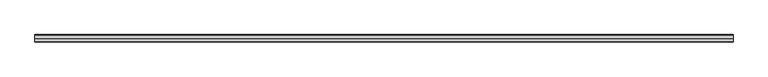
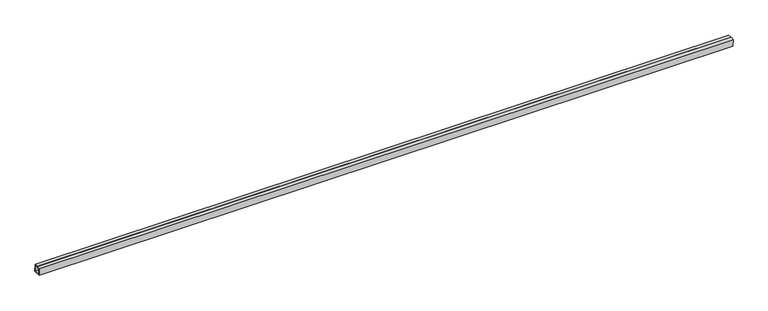
"""IFC4 building model written with IfcOpenShell, lengths in millimetres: proxy geometry, Inner panel:Inner panel:1:Inner panel:1 : Inner panel:Inner panel:300324:2:Inner panel:1:Inner panel:1 : Inner panel:Inner panel:300324:2 : Inner panel:Inner panel:1:Inner panel:1 : Inner panel:Inner panel:300324:300043:2 : Inner panel:Inner panel:1:Inner panel:1 : Inner panel:Inner panel:300324:2:Inner panel:1:Inner panel:1 : Inner panel:Inner panel:300324:2 : Inner panel:Inner panel:1:Inner panel:1 : Inner panel:Inner panel:300324:300043:308120."""

import ifcopenshell
import ifcopenshell.guid

model = None  # the IFC model being written
_history = None  # IfcOwnerHistory: only IFC2X3 demands one
_inside = {}  # id of a spatial element -> (the spatial element, [elements in it])
_under = {}  # id of a project, library or spatial element -> (it, [spatial elements below it])
_declared = {}  # id of a project -> (the project, [libraries it declares])
_typed = {}  # id of a type object -> (the type object, [elements of that type])
_made_of = {}  # id of a material, layer set ... -> (it, [elements and type objects made of it])


def new_model(schema):
    """Start an empty IFC model of exactly this schema.

    Asked for "IFC4X3", IfcOpenShell would pick the latest addendum, in which some entities
    have other attributes; the version numbers below select the first issue.
    IFC2X3 requires an IfcOwnerHistory on every rooted entity: one is made here for all.
    """
    global model, _history
    if schema == "IFC4X3":
        model = ifcopenshell.file(schema_version=(4, 3, 0, 0))
    else:
        model = ifcopenshell.file(schema=schema)
    _inside.clear()
    _under.clear()
    _declared.clear()
    _typed.clear()
    _made_of.clear()
    _history = None
    if model.schema == "IFC2X3":
        org = make("IfcOrganization", Name="unknown")
        user = make(
            "IfcPersonAndOrganization",
            ThePerson=make("IfcPerson", FamilyName="unknown"),
            TheOrganization=org,
        )
        app = make(
            "IfcApplication",
            ApplicationDeveloper=org,
            Version="unknown",
            ApplicationFullName="unknown",
            ApplicationIdentifier="unknown",
        )
        _history = make(
            "IfcOwnerHistory",
            OwningUser=user,
            OwningApplication=app,
            ChangeAction="ADDED",
            CreationDate=0,
        )
    return model


def make(cls, **values):
    """One entity of the class cls with the attributes given. An attribute that is None is left unset."""
    return model.create_entity(
        cls, **{name: value for name, value in values.items() if value is not None}
    )


def rooted(cls, **values):
    """An entity with a GlobalId (a new one), such as an element, a storey or a relation."""
    return make(cls, GlobalId=ifcopenshell.guid.new(), OwnerHistory=_history, **values)


def si_unit(unit_type, name, prefix=None):
    """IfcSIUnit, for example si_unit("LENGTHUNIT", "METRE", prefix="MILLI")."""
    return make("IfcSIUnit", UnitType=unit_type, Prefix=prefix, Name=name)


def assignment(units):
    """IfcUnitAssignment: the units of a project."""
    return None if units is None else make("IfcUnitAssignment", Units=units)


def point(xyz):
    """IfcCartesianPoint."""
    return None if xyz is None else make("IfcCartesianPoint", Coordinates=xyz)


def direction(xyz):
    """IfcDirection."""
    return None if xyz is None else make("IfcDirection", DirectionRatios=xyz)


def frame(location, z_axis=None, x_axis=None):
    """IfcAxis2Placement3D, a coordinate frame: its origin and axes. An axis left out is left unset."""
    return make(
        "IfcAxis2Placement3D",
        Location=point(location),
        Axis=direction(z_axis),
        RefDirection=direction(x_axis),
    )


def origin():
    """The frame at (0, 0, 0) with its axes left unset."""
    return frame((0.0, 0.0, 0.0))


def place(relative_to, where):
    """IfcLocalPlacement: puts the frame where relative to a parent placement (None: the world)."""
    return make(
        "IfcLocalPlacement", PlacementRelTo=relative_to, RelativePlacement=where
    )


def context(
    kind, dimensions, precision=None, world=None, true_north=None, identifier=None
):
    """IfcGeometricRepresentationContext, for example the 3D "Model" context."""
    return make(
        "IfcGeometricRepresentationContext",
        ContextIdentifier=identifier,
        ContextType=kind,
        CoordinateSpaceDimension=dimensions,
        Precision=precision,
        WorldCoordinateSystem=world,
        TrueNorth=true_north,
    )


def project(units=None, contexts=None):
    """IfcProject with its units and contexts."""
    return rooted(
        "IfcProject",
        Name="project",
        RepresentationContexts=contexts,
        UnitsInContext=assignment(units),
    )


def spatial(cls, under=None, at=None, **own):
    """A site, building, storey or space (cls), placed at a placement, below another one or the project."""
    s = rooted(cls, ObjectPlacement=at, **own)
    if under is not None:
        _under.setdefault(under.id(), (under, []))[1].append(s)
    return s


def polyline(points):
    """IfcPolyline through the points."""
    return make("IfcPolyline", Points=[point(p) for p in points])


def outline(outer, holes=None, kind="AREA"):
    """IfcArbitraryClosedProfileDef: a profile drawn as a closed curve; with holes, ...WithVoids."""
    if holes is None:
        return make("IfcArbitraryClosedProfileDef", ProfileType=kind, OuterCurve=outer)
    return make(
        "IfcArbitraryProfileDefWithVoids",
        ProfileType=kind,
        OuterCurve=outer,
        InnerCurves=holes,
    )


def extrude(swept, where, along, depth):
    """IfcExtrudedAreaSolid: the profile swept, set in the frame where, extruded along a direction by depth."""
    return make(
        "IfcExtrudedAreaSolid",
        SweptArea=swept,
        Position=where,
        ExtrudedDirection=direction(along),
        Depth=depth,
    )


def shape(context_of_items, identifier, shape_type, items):
    """IfcShapeRepresentation: the items that make up one representation, for example the "Body"."""
    return make(
        "IfcShapeRepresentation",
        ContextOfItems=context_of_items,
        RepresentationIdentifier=identifier,
        RepresentationType=shape_type,
        Items=items,
    )


def source(mapping_origin, context_of_items, identifier, shape_type, items):
    """IfcRepresentationMap: a shape defined once, which mapped items show again and again."""
    return make(
        "IfcRepresentationMap",
        MappingOrigin=mapping_origin,
        MappedRepresentation=shape(context_of_items, identifier, shape_type, items),
    )


def transform(
    local_origin,
    x_axis=None,
    y_axis=None,
    z_axis=None,
    scale=None,
    scale2=None,
    scale3=None,
    uniform=True,
):
    """IfcCartesianTransformationOperator3D, or its non-uniform kind. x_axis, y_axis, z_axis: its Axis1, 2, 3."""
    if uniform:
        return make(
            "IfcCartesianTransformationOperator3D",
            Axis1=direction(x_axis),
            Axis2=direction(y_axis),
            LocalOrigin=point(local_origin),
            Scale=scale,
            Axis3=direction(z_axis),
        )
    return make(
        "IfcCartesianTransformationOperator3DnonUniform",
        Axis1=direction(x_axis),
        Axis2=direction(y_axis),
        LocalOrigin=point(local_origin),
        Scale=scale,
        Axis3=direction(z_axis),
        Scale2=scale2,
        Scale3=scale3,
    )


def mapped(mapping_source, mapping_target):
    """IfcMappedItem: shows the shape of a source again, moved by a transform."""
    return make(
        "IfcMappedItem", MappingSource=mapping_source, MappingTarget=mapping_target
    )


def made_of(thing, what):
    """Note that an element or type object is made of a material, layer set ...; save() writes the relation."""
    if what is not None:
        _made_of.setdefault(what.id(), (what, []))[1].append(thing)
    return thing


def element(
    cls,
    number,
    at=None,
    inside=None,
    cuts=None,
    type_object=None,
    material=None,
    context=None,
    identifier="Body",
    shape_type=None,
    held_by="IfcProductDefinitionShape",
    body=None,
    shapes=None,
    **own,
):
    """One element of the class cls, such as IfcWall. Its Tag is "e" and its number.

    at: its placement. inside: the storey or other place that contains it. cuts: it is an
    opening in that element (IfcRelVoidsElement). A single representation is given by context,
    identifier, shape_type and body (its items); several are given by shapes. held_by: the class
    of the entity that holds the representations. save() writes the other relations.
    """
    e = rooted(cls, Tag="e%d" % number, ObjectPlacement=at, **own)
    if body is not None:
        shapes = [shape(context, identifier, shape_type, body)]
    if shapes is not None:
        e.Representation = make(held_by, Representations=shapes)
    if inside is not None:
        _inside.setdefault(inside.id(), (inside, []))[1].append(e)
    if cuts is not None:
        rooted(
            "IfcRelVoidsElement", RelatingBuildingElement=cuts, RelatedOpeningElement=e
        )
    if type_object is not None:
        _typed.setdefault(type_object.id(), (type_object, []))[1].append(e)
    return made_of(e, material)


def aggregate(whole, parts):
    """IfcRelAggregates: a whole, such as a stair, and the parts it consists of."""
    return rooted("IfcRelAggregates", RelatingObject=whole, RelatedObjects=parts)


def save(model, path):
    """Write the relations noted so far, then the file.

    IfcRelAggregates (storeys below a building ...), IfcRelContainedInSpatialStructure (elements
    in a storey), IfcRelDefinesByType, IfcRelAssociatesMaterial and IfcRelDeclares: one each for
    every whole, place, type object, material and project.
    """
    for whole, parts in _under.values():
        aggregate(whole, parts)
    for where, things in _inside.values():
        rooted(
            "IfcRelContainedInSpatialStructure",
            RelatedElements=things,
            RelatingStructure=where,
        )
    for kind, things in _typed.values():
        rooted("IfcRelDefinesByType", RelatedObjects=things, RelatingType=kind)
    for what, things in _made_of.values():
        rooted("IfcRelAssociatesMaterial", RelatedObjects=things, RelatingMaterial=what)
    for by, libraries in _declared.values():
        rooted("IfcRelDeclares", RelatingContext=by, RelatedDefinitions=libraries)
    model.write(path)


def generic_models_22e957f1(model_context):
    return source(origin(), model_context, "Body", "SweptSolid", [
        extrude(outline(polyline([(-579878.6983883, 3913.3147263), (-579860.4579651, 3914.0747439), (-579858.8718413, 3876.0077738), (-579896.9388114, 3874.4216501), (-579898.5249352, 3912.4886201), (-579880.284512, 3913.2486378), (-579880.1853793, 3910.8694521), (-579896.0466168, 3910.2085672), (-579894.6587585, 3876.8999684), (-579861.3501597, 3878.2878267), (-579862.738018, 3911.5964255), (-579878.5992555, 3910.9355406), (-579878.6983883, 3913.3147263)])), frame((593141.1867239, 0.0, 0.0), z_axis=(1.0, 0.0, 0.0), x_axis=(0.0, 1.0, 0.0)), (0.0, 0.0, 1.0), 3657.6),
    ])


if __name__ == "__main__":
    model = new_model("IFC4")
    model_context = context("Model", 3, world=origin())
    ifc_project = project(units=[si_unit("LENGTHUNIT", "METRE", prefix="MILLI")], contexts=[model_context])
    site = spatial("IfcSite", under=ifc_project)
    building = spatial("IfcBuilding", under=site)
    placement = place(None, origin())
    generic_models_shape = generic_models_22e957f1(model_context)
    element("IfcBuildingElementProxy", 1, Name="Inner panel:Inner panel:1:Inner panel:1 : Inner panel:Inner panel:300324:2:Inner panel:1:Inner panel:1 : Inner panel:Inner panel:300324:2 : Inner panel:Inner panel:1:Inner panel:1 : Inner panel:Inner panel:300324:300043:2 : Inner panel:Inner panel:1:Inner panel:1 : Inner panel:Inner panel:300324:2:Inner panel:1:Inner panel:1 : Inner panel:Inner panel:300324:2 : Inner panel:Inner panel:1:Inner panel:1 : Inner panel:Inner panel:300324:300043:308120", ObjectType="Inner panel:Inner panel:1:Inner panel:1 : Inner panel:Inner panel:300324:2:Inner panel:1:Inner panel:1 : Inner panel:Inner panel:300324:2 : Inner panel:Inner panel:1:Inner panel:1 : Inner panel:Inner panel:300324:300043:2 : Inner panel:Inner panel:1:Inner panel:1 : Inner panel:Inner panel:300324:2:Inner panel:1:Inner panel:1 : Inner panel:Inner panel:300324:2 : Inner panel:Inner panel:1:Inner panel:1 : Inner panel:Inner panel:300324:300043:308120", at=placement, inside=building, context=model_context, shape_type="MappedRepresentation", body=[
        mapped(generic_models_shape, transform((0.0, 0.0, 0.0), x_axis=(1.0, 0.0, 0.0), y_axis=(0.0, 1.0, 0.0), z_axis=(0.0, 0.0, 1.0))),
    ])
    save(model, "model.ifc")

# Revit data of these elements
# Type "Inner panel:Inner panel:1:Inner panel:1 : Inner panel:Inner panel:300324:2:Inner panel:1:Inner panel:1 : Inner panel:Inner panel:300324:2 : Inner panel:Inner panel:1:Inner panel:1 : Inner panel:Inner panel:300324:300043:2 : Inner panel:Inner panel:1:Inner panel:1 : Inner panel:Inner panel:300324:2:Inner panel:1:Inner panel:1 : Inner panel:Inner panel:300324:2 : Inner panel:Inner panel:1:Inner panel:1 : Inner panel:Inner panel:300324:300043:308120"
#   NameOverride = "Inner panel:Inner panel:1:Inner panel:1 : Inner panel:Inner panel:300324:2:Inner panel:1:Inner panel:1 : Inner panel:Inner panel:300324:2 : Inner panel:Inner panel:1:Inner panel:1 : Inner panel:Inner panel:300324:300043:308120"
#   ObjectTypeOverride = "Inner panel:1:Inner panel:1 : Inner panel:Inner panel:300324:2 : Inner panel:Inner panel:1:Inner panel:1 : Inner panel:Inner panel:300324:300043"
#   Reference = "Inner panel"
#   Tag = "308120"
# Element 1 (IfcBuildingElementProxy, "Inner panel:Inner panel:1:Inner panel:1 : Inner panel:Inner panel:300324:2:Inner panel:1:Inner panel:1 : Inner panel:Inner panel:300324:2 : Inner panel:Inner panel:1:Inner panel:1 : Inner panel:Inner panel:300324:300043:2 : Inner panel:Inner panel:1:Inner panel:1 : Inner panel:Inner panel:300324:2:Inner panel:1:Inner panel:1 : Inner panel:Inner panel:300324:2 : Inner panel:Inner panel:1:Inner panel:1 : Inner panel:Inner panel:300324:300043:308120")
#   Materials on its faces: "1 1/2\" X 1 1/2\" SPLIT-SEAM SQUARE TUBING (~24\" CANTILEVER FROM C.L. OF GLULAM)"
# Materials
#   "1 1/2\" X 1 1/2\" SPLIT-SEAM SQUARE TUBING (~24\" CANTILEVER FROM C.L. OF GLULAM)": class "Unassigned", colour RGB 202 201 200, transparency 0, Cost = 0
